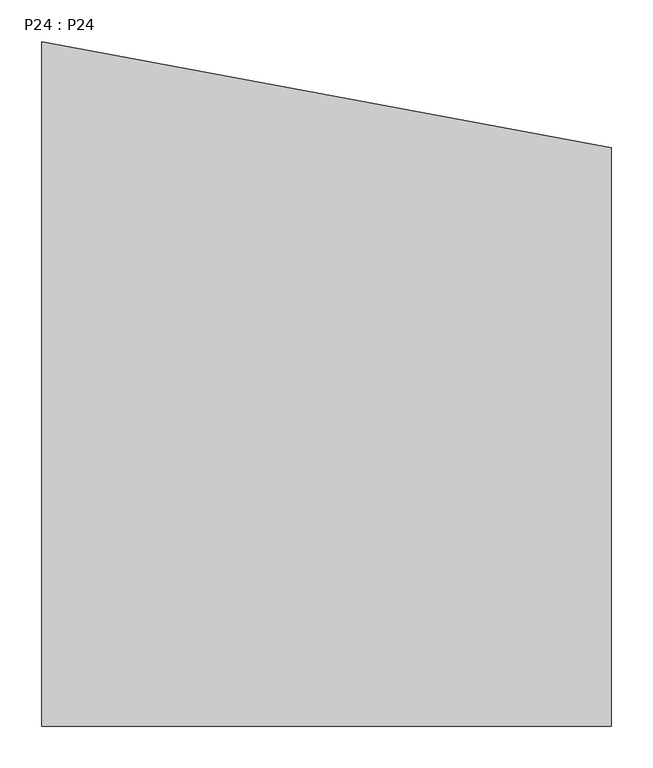
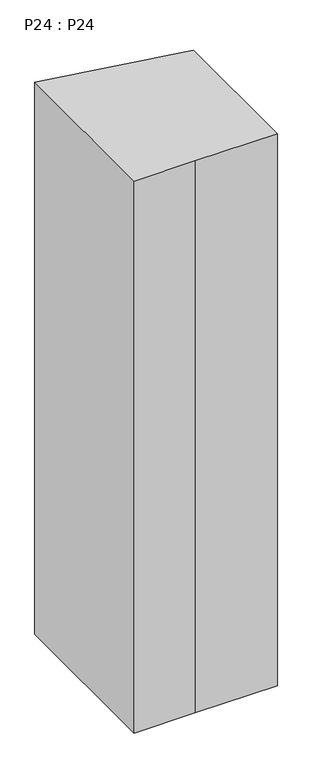
"""IFC4 building model written with IfcOpenShell, lengths in millimetres: column geometry, P24 : P24."""

from ifc_helpers import new_model, si_unit, frame, origin, place, context, project, spatial, polyline, outline, extrude, source, transform, mapped, element, save


def p24_p24_21724a61(model_context):
    return source(origin(), model_context, "Body", "SweptSolid", [
        extrude(outline(polyline([(393.7, 21245.0916402), (393.7, 20548.6), (0.0, 20548.6), (-292.1, 20548.6), (-292.1, 21372.919497), (393.7, 21245.0916402)])), frame((0.0, 0.0, 8756.65), z_axis=(0.0, 0.0, 1.0), x_axis=(1.0, 0.0, 0.0)), (0.0, 0.0, 1.0), 2794.0),
    ])


if __name__ == "__main__":
    model = new_model("IFC4")
    model_context = context("Model", 3, world=origin())
    ifc_project = project(units=[si_unit("LENGTHUNIT", "METRE", prefix="MILLI")], contexts=[model_context])
    site = spatial("IfcSite", under=ifc_project)
    building = spatial("IfcBuilding", under=site)
    placement = place(None, origin())
    p24_p24_shape = p24_p24_21724a61(model_context)
    element("IfcColumn", 1, ObjectType="P24 : P24", at=placement, inside=building, context=model_context, shape_type="MappedRepresentation", body=[
        mapped(p24_p24_shape, transform((0.0, 0.0, 0.0), x_axis=(1.0, 0.0, 0.0), y_axis=(0.0, 1.0, 0.0), z_axis=(0.0, 0.0, 1.0))),
    ])
    save(model, "model.ifc")

# Revit data of these elements
# Type "P24 : P24"
#   Type Mark = "P24"
# Element 1 (IfcColumn, "P24 : P24")
#   Materials on its faces: "16 - Concrete - Cast-in-Place"
# Materials
#   "16 - Concrete - Cast-in-Place": class "Unassigned", colour RGB 192 192 192, transparency 0, Description = "Concrete", Cost = 0
